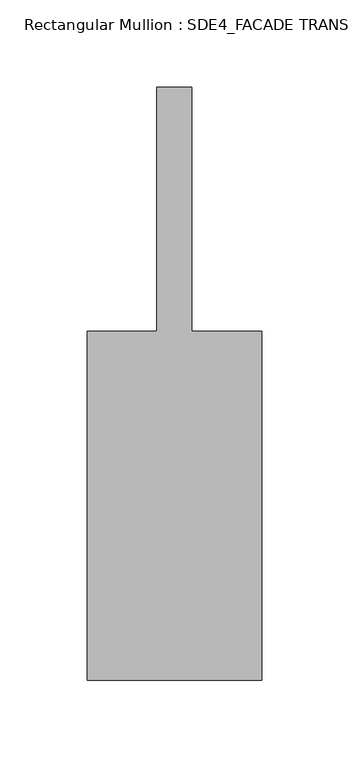
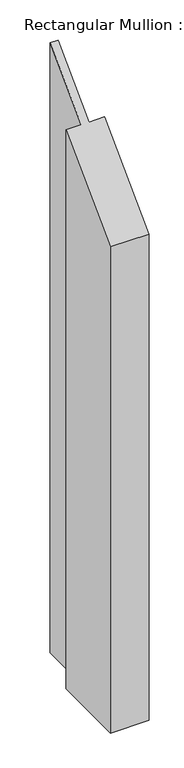
"""IFC4 building model written with IfcOpenShell, lengths in millimetres: member geometry, Rectangular Mullion : SDE4_FACADE TRANSOM TYPE 1."""

from ifc_helpers import new_model, si_unit, origin, place, context, project, spatial, faceted_brep, source, transform, mapped, element, save


def rectangular_mullion_sde4_facade_transom_type_1_553cd024(model_context):
    return source(origin(), model_context, "Body", "Brep", [
        faceted_brep([(50.0, -132.5, -1466.4475465), (-50.0, -132.5, -1466.4475465), (-50.0, 67.5, -1466.4475465), (-10.0, 67.5, -1466.4475465), (-10.0, 207.5, -1466.4475465), (10.0, 207.5, -1466.4475465), (10.0, 67.5, -1466.4475465), (50.0, 67.5, -1466.4475465), (50.0, 67.5, 67.5), (50.0, -132.5, -132.5), (10.0, 67.5, 67.5), (10.0, 207.5, 207.5), (-10.0, 207.5, 207.5), (-10.0, 67.5, 67.5), (-50.0, 67.5, 67.5), (-50.0, -132.5, -132.5)], [[[0, 1, 2, 3, 4, 5, 6, 7]], [[8, 9, 0, 7]], [[10, 8, 7, 6]], [[11, 10, 6, 5]], [[12, 11, 5, 4]], [[13, 12, 4, 3]], [[14, 13, 3, 2]], [[15, 14, 2, 1]], [[9, 15, 1, 0]], [[9, 8, 10, 11, 12, 13, 14, 15]]]),
    ])


if __name__ == "__main__":
    model = new_model("IFC4")
    model_context = context("Model", 3, world=origin())
    ifc_project = project(units=[si_unit("LENGTHUNIT", "METRE", prefix="MILLI")], contexts=[model_context])
    site = spatial("IfcSite", under=ifc_project)
    building = spatial("IfcBuilding", under=site)
    placement = place(None, origin())
    rectangular_mullion_sde4_facade_transom_type_1_shape = rectangular_mullion_sde4_facade_transom_type_1_553cd024(model_context)
    element("IfcMember", 1, ObjectType="Rectangular Mullion : SDE4_FACADE TRANSOM TYPE 1", at=placement, inside=building, context=model_context, shape_type="MappedRepresentation", body=[
        mapped(rectangular_mullion_sde4_facade_transom_type_1_shape, transform((0.0, 0.0, 0.0), x_axis=(1.0, 0.0, 0.0), y_axis=(0.0, 1.0, 0.0), z_axis=(0.0, 0.0, 1.0))),
    ])
    save(model, "model.ifc")

# Revit data of these elements
# Type "Rectangular Mullion : SDE4_FACADE TRANSOM TYPE 1"
#   built-in parameter 1007322 = 1.11549 (stored number, unit not read)
#   built-in parameter 1007321 = 0.164042 (stored number, unit not read)
#   built-in parameter 1007320 = 0.164042 (stored number, unit not read)
